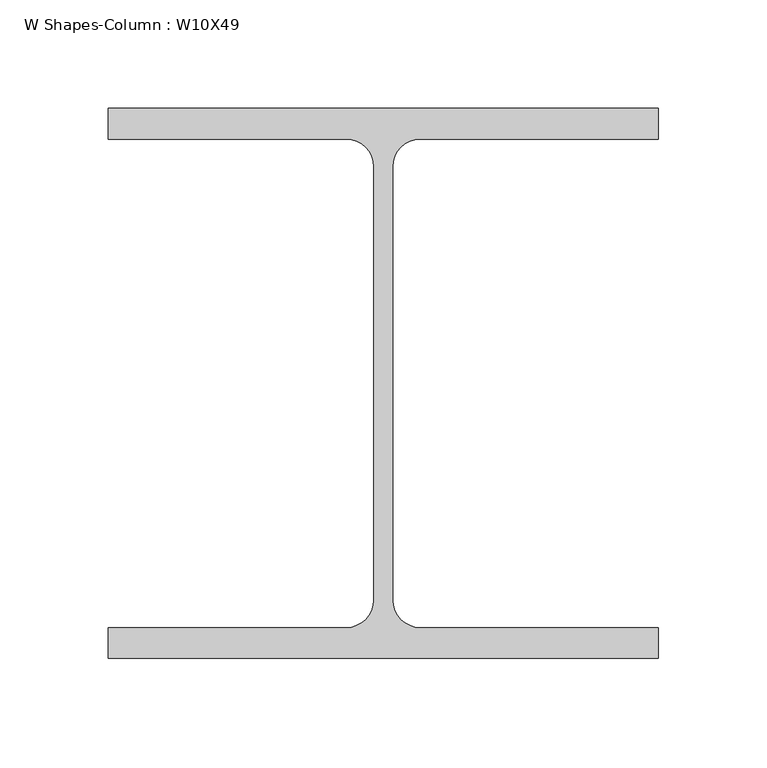
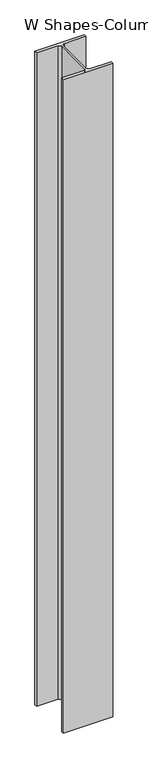
"""IFC4 building model written with IfcOpenShell, lengths in millimetres: column geometry, W Shapes-Column : W10X49."""

from ifc_helpers import new_model, si_unit, point, frame, frame_2d, origin, place, context, project, spatial, polyline, circle_curve, trimmed, segment, composite_curve, outline, extrude, source, transform, mapped, element, save


def w_shapes_column_w10x49_39fde8e9(model_context):
    return source(origin(), model_context, "Body", "SweptSolid", [
        extrude(outline(composite_curve([segment(polyline([(127.0, 127.0), (127.0, 112.776), (17.018, 112.776)]), True, "CONTINUOUS"), segment(trimmed(circle_curve(frame_2d((17.018, 100.076)), 12.7), [point((17.018, 112.776))], [point((4.318, 100.076))], True, "CARTESIAN"), True, "CONTINUOUS"), segment(polyline([(4.318, 100.076), (4.318, -100.076)]), True, "CONTINUOUS"), segment(trimmed(circle_curve(frame_2d((17.018, -100.076)), 12.7), [point((4.318, -100.076))], [point((17.018, -112.776))], True, "CARTESIAN"), True, "CONTINUOUS"), segment(polyline([(17.018, -112.776), (127.0, -112.776), (127.0, -127.0), (-127.0, -127.0), (-127.0, -112.776), (-17.018, -112.776)]), True, "CONTINUOUS"), segment(trimmed(circle_curve(frame_2d((-17.018, -100.076)), 12.7), [point((-17.018, -112.776))], [point((-4.318, -100.076))], True, "CARTESIAN"), True, "CONTINUOUS"), segment(polyline([(-4.318, -100.076), (-4.318, 100.076)]), True, "CONTINUOUS"), segment(trimmed(circle_curve(frame_2d((-17.018, 100.076)), 12.7), [point((-4.318, 100.076))], [point((-17.018, 112.776))], True, "CARTESIAN"), True, "CONTINUOUS"), segment(polyline([(-17.018, 112.776), (-127.0, 112.776), (-127.0, 127.0), (127.0, 127.0)]), True, "CONTINUOUS")], self_intersect=False)), frame((0.0, 0.0, -3556.0), z_axis=(0.0, 0.0, 1.0), x_axis=(1.0, 0.0, 0.0)), (0.0, 0.0, 1.0), 3556.0),
    ])


if __name__ == "__main__":
    model = new_model("IFC4")
    model_context = context("Model", 3, world=origin())
    ifc_project = project(units=[si_unit("LENGTHUNIT", "METRE", prefix="MILLI")], contexts=[model_context])
    site = spatial("IfcSite", under=ifc_project)
    building = spatial("IfcBuilding", under=site)
    placement = place(None, origin())
    w_shapes_column_w10x49_shape = w_shapes_column_w10x49_39fde8e9(model_context)
    element("IfcColumn", 1, ObjectType="W Shapes-Column : W10X49", at=placement, inside=building, context=model_context, shape_type="MappedRepresentation", body=[
        mapped(w_shapes_column_w10x49_shape, transform((0.0, 0.0, 0.0), x_axis=(1.0, 0.0, 0.0), y_axis=(0.0, 1.0, 0.0), z_axis=(0.0, 0.0, 1.0))),
    ])
    save(model, "model.ifc")

# Revit data of these elements
# Type "W Shapes-Column : W10X49"
#   COBie.Type.CreatedBy = "doug.wood@us.ibm.com"
#   COBie.Type.CreatedOn = "2016-04-14T02:07:24"
#   COBie.Type.Name = "Structural Columns_W Shapes-Column_W10X49"
#   COBie.Type.Category = "23-25 30 11 14 11 : Columns"
#   COBie.Type.Description = "W Shapes-Column_W10X49"
#   COBie.Type.Manufacturer = ""
#   COBie.Type.ModelNumber = ""
#   Section Name Key = "W10x49"
#   Assembly Code = "B10"
#   COBie.Type.ReplacementCost = 0
#   Width = 254 mm
#   Web Thickness = 8.636 mm
#   Web Fillet = 12.7 mm
#   Warping Constant = 555869.2 cm⁶
#   Torsional Moment of Inertia = 57.8562 cm⁴
#   Section Area = 14.40 in²
#   Plastic Modulus weak axis = 0.0163773 (stored number, unit not read)
#   Plastic Modulus strong axis = 0.0349537 (stored number, unit not read)
#   Perimeter = 17.8308 m²/m
#   Nominal Weight = 715.101 N/m
#   Moment of Inertia weak axis = 3887.6 cm⁴
#   Moment of Inertia strong axis = 11321.5 cm⁴
#   Height = 254 mm
#   Flange Thickness = 14.224 mm
#   Elastic Modulus weak axis = 0.0108218 (stored number, unit not read)
#   Elastic Modulus strong axis = 0.0315972 (stored number, unit not read)
#   Centroid Vertical = 127 mm
#   Centroid Horizontal = 127 mm
#   COBie.Type = no
#   Structural Material [instance default] = Steel ASTM A992
#   Principal Axes Angle = 0
# Element 1 (IfcColumn, "W Shapes-Column : W10X49")
#   Materials on its faces: "Steel ASTM A992"
# Materials
#   "Steel ASTM A992": class "Metal", colour RGB 199 199 199, transparency 0, Description = "Structural steel 50ksi", Cost = 0
